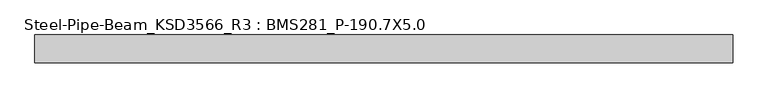
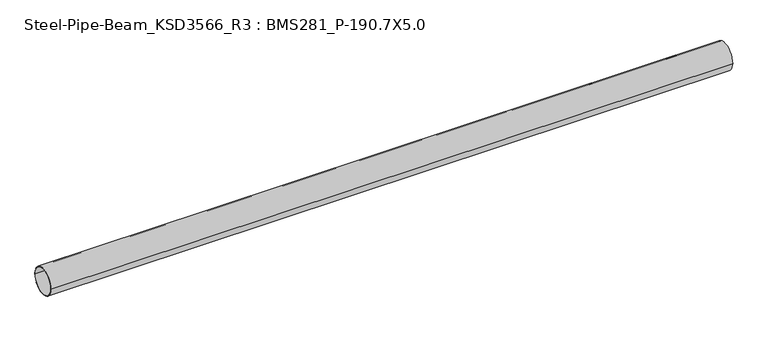
"""IFC4 building model written with IfcOpenShell, lengths in millimetres: member geometry, Steel-Pipe-Beam_KSD3566_R3 : BMS281_P-190.7X5.0."""

from ifc_helpers import new_model, si_unit, point, frame, origin, origin_2d, place, context, project, spatial, circle_curve, trimmed, segment, composite_curve, outline, extrude, source, transform, mapped, element, save


def steel_pipe_beam_ksd3566_r3_bms281_p_190_7x5_0_d6fb346a(model_context):
    return source(origin(), model_context, "Body", "SweptSolid", [
        extrude(outline(composite_curve([segment(trimmed(circle_curve(origin_2d(), 95.35), [point((-95.35, 0.0))], [point((95.35, 0.0))], False, "CARTESIAN"), True, "CONTINUOUS"), segment(trimmed(circle_curve(origin_2d(), 95.35), [point((95.35, 0.0))], [point((-95.35, 0.0))], False, "CARTESIAN"), True, "CONTINUOUS")], self_intersect=False), holes=[composite_curve([segment(trimmed(circle_curve(origin_2d(), 90.35), [point((90.35, 0.0))], [point((-90.35, 0.0))], True, "CARTESIAN"), True, "CONTINUOUS"), segment(trimmed(circle_curve(origin_2d(), 90.35), [point((-90.35, 0.0))], [point((90.35, 0.0))], True, "CARTESIAN"), True, "CONTINUOUS")], self_intersect=False)]), frame((-2413.1370429, 0.0, 0.0), z_axis=(1.0, 0.0, 0.0), x_axis=(0.0, 1.0, 0.0)), (0.0, 0.0, 1.0), 4740.8627767),
    ])


if __name__ == "__main__":
    model = new_model("IFC4")
    model_context = context("Model", 3, world=origin())
    ifc_project = project(units=[si_unit("LENGTHUNIT", "METRE", prefix="MILLI")], contexts=[model_context])
    site = spatial("IfcSite", under=ifc_project)
    building = spatial("IfcBuilding", under=site)
    placement = place(None, origin())
    steel_pipe_beam_ksd3566_r3_bms281_p_190_7x5_0_shape = steel_pipe_beam_ksd3566_r3_bms281_p_190_7x5_0_d6fb346a(model_context)
    element("IfcMember", 1, ObjectType="Steel-Pipe-Beam_KSD3566_R3 : BMS281_P-190.7X5.0", at=placement, inside=building, context=model_context, shape_type="MappedRepresentation", body=[
        mapped(steel_pipe_beam_ksd3566_r3_bms281_p_190_7x5_0_shape, transform((0.0, 0.0, 0.0), x_axis=(1.0, 0.0, 0.0), y_axis=(0.0, 1.0, 0.0), z_axis=(0.0, 0.0, 1.0))),
    ])
    save(model, "model.ifc")

# Revit data of these elements
# Type "Steel-Pipe-Beam_KSD3566_R3 : BMS281_P-190.7X5.0"
#   Keynote = "P-190.7X5.0"
#   SteelWeight = "Light"
#   t = 0.0050 m
#   Surface Area = 0.599102 m²/m
#   Section Area = 29.1697 cm²
#   Mass per Unit Length = 22.8982 kg/m
#   Length [instance default] = 1.5000 m
#   D = 0.1907 m
#   hec_material4 [instance default] = none
#   hec_material3 [instance default] = none
#   hec_material2 [instance default] = none
#   hec_material1 [instance default] = none
#   Structural Material [instance default] = Steel, 45-345
#   Assembly Code = ""
# Element 1 (IfcMember, "Steel-Pipe-Beam_KSD3566_R3 : BMS281_P-190.7X5.0")
#   Structural Material = none
# Materials
#   "Steel, 45-345": class "Metal", colour RGB 189 187 185, transparency 0, Description = "Steel 345 MPa", Cost = 0
